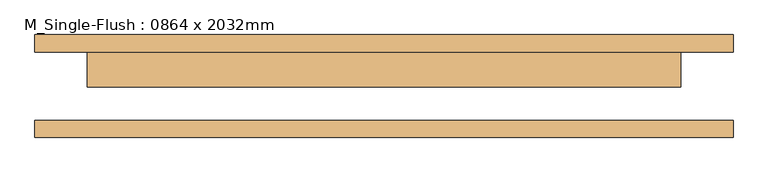
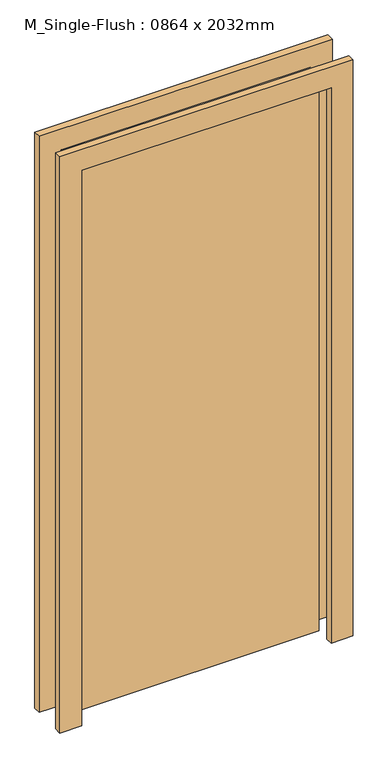
"""IFC4 building model written with IfcOpenShell, lengths in millimetres: door geometry, M_Single-Flush : 0864 x 2032mm."""

import ifcopenshell
import ifcopenshell.guid

model = None  # the IFC model being written
_history = None  # IfcOwnerHistory: only IFC2X3 demands one
_inside = {}  # id of a spatial element -> (the spatial element, [elements in it])
_under = {}  # id of a project, library or spatial element -> (it, [spatial elements below it])
_declared = {}  # id of a project -> (the project, [libraries it declares])
_typed = {}  # id of a type object -> (the type object, [elements of that type])
_made_of = {}  # id of a material, layer set ... -> (it, [elements and type objects made of it])


def new_model(schema):
    """Start an empty IFC model of exactly this schema.

    Asked for "IFC4X3", IfcOpenShell would pick the latest addendum, in which some entities
    have other attributes; the version numbers below select the first issue.
    IFC2X3 requires an IfcOwnerHistory on every rooted entity: one is made here for all.
    """
    global model, _history
    if schema == "IFC4X3":
        model = ifcopenshell.file(schema_version=(4, 3, 0, 0))
    else:
        model = ifcopenshell.file(schema=schema)
    _inside.clear()
    _under.clear()
    _declared.clear()
    _typed.clear()
    _made_of.clear()
    _history = None
    if model.schema == "IFC2X3":
        org = make("IfcOrganization", Name="unknown")
        user = make(
            "IfcPersonAndOrganization",
            ThePerson=make("IfcPerson", FamilyName="unknown"),
            TheOrganization=org,
        )
        app = make(
            "IfcApplication",
            ApplicationDeveloper=org,
            Version="unknown",
            ApplicationFullName="unknown",
            ApplicationIdentifier="unknown",
        )
        _history = make(
            "IfcOwnerHistory",
            OwningUser=user,
            OwningApplication=app,
            ChangeAction="ADDED",
            CreationDate=0,
        )
    return model


def make(cls, **values):
    """One entity of the class cls with the attributes given. An attribute that is None is left unset."""
    return model.create_entity(
        cls, **{name: value for name, value in values.items() if value is not None}
    )


def rooted(cls, **values):
    """An entity with a GlobalId (a new one), such as an element, a storey or a relation."""
    return make(cls, GlobalId=ifcopenshell.guid.new(), OwnerHistory=_history, **values)


def si_unit(unit_type, name, prefix=None):
    """IfcSIUnit, for example si_unit("LENGTHUNIT", "METRE", prefix="MILLI")."""
    return make("IfcSIUnit", UnitType=unit_type, Prefix=prefix, Name=name)


def assignment(units):
    """IfcUnitAssignment: the units of a project."""
    return None if units is None else make("IfcUnitAssignment", Units=units)


def point(xyz):
    """IfcCartesianPoint."""
    return None if xyz is None else make("IfcCartesianPoint", Coordinates=xyz)


def direction(xyz):
    """IfcDirection."""
    return None if xyz is None else make("IfcDirection", DirectionRatios=xyz)


def frame(location, z_axis=None, x_axis=None):
    """IfcAxis2Placement3D, a coordinate frame: its origin and axes. An axis left out is left unset."""
    return make(
        "IfcAxis2Placement3D",
        Location=point(location),
        Axis=direction(z_axis),
        RefDirection=direction(x_axis),
    )


def origin():
    """The frame at (0, 0, 0) with its axes left unset."""
    return frame((0.0, 0.0, 0.0))


def origin_with_axes():
    """The frame at (0, 0, 0) with the z axis (0, 0, 1) and the x axis (1, 0, 0) written out."""
    return frame((0.0, 0.0, 0.0), z_axis=(0.0, 0.0, 1.0), x_axis=(1.0, 0.0, 0.0))


def place(relative_to, where):
    """IfcLocalPlacement: puts the frame where relative to a parent placement (None: the world)."""
    return make(
        "IfcLocalPlacement", PlacementRelTo=relative_to, RelativePlacement=where
    )


def context(
    kind, dimensions, precision=None, world=None, true_north=None, identifier=None
):
    """IfcGeometricRepresentationContext, for example the 3D "Model" context."""
    return make(
        "IfcGeometricRepresentationContext",
        ContextIdentifier=identifier,
        ContextType=kind,
        CoordinateSpaceDimension=dimensions,
        Precision=precision,
        WorldCoordinateSystem=world,
        TrueNorth=true_north,
    )


def project(units=None, contexts=None):
    """IfcProject with its units and contexts."""
    return rooted(
        "IfcProject",
        Name="project",
        RepresentationContexts=contexts,
        UnitsInContext=assignment(units),
    )


def spatial(cls, under=None, at=None, **own):
    """A site, building, storey or space (cls), placed at a placement, below another one or the project."""
    s = rooted(cls, ObjectPlacement=at, **own)
    if under is not None:
        _under.setdefault(under.id(), (under, []))[1].append(s)
    return s


def polyline(points):
    """IfcPolyline through the points."""
    return make("IfcPolyline", Points=[point(p) for p in points])


def outline(outer, holes=None, kind="AREA"):
    """IfcArbitraryClosedProfileDef: a profile drawn as a closed curve; with holes, ...WithVoids."""
    if holes is None:
        return make("IfcArbitraryClosedProfileDef", ProfileType=kind, OuterCurve=outer)
    return make(
        "IfcArbitraryProfileDefWithVoids",
        ProfileType=kind,
        OuterCurve=outer,
        InnerCurves=holes,
    )


def extrude(swept, where, along, depth):
    """IfcExtrudedAreaSolid: the profile swept, set in the frame where, extruded along a direction by depth."""
    return make(
        "IfcExtrudedAreaSolid",
        SweptArea=swept,
        Position=where,
        ExtrudedDirection=direction(along),
        Depth=depth,
    )


def shape(context_of_items, identifier, shape_type, items):
    """IfcShapeRepresentation: the items that make up one representation, for example the "Body"."""
    return make(
        "IfcShapeRepresentation",
        ContextOfItems=context_of_items,
        RepresentationIdentifier=identifier,
        RepresentationType=shape_type,
        Items=items,
    )


def source(mapping_origin, context_of_items, identifier, shape_type, items):
    """IfcRepresentationMap: a shape defined once, which mapped items show again and again."""
    return make(
        "IfcRepresentationMap",
        MappingOrigin=mapping_origin,
        MappedRepresentation=shape(context_of_items, identifier, shape_type, items),
    )


def transform(
    local_origin,
    x_axis=None,
    y_axis=None,
    z_axis=None,
    scale=None,
    scale2=None,
    scale3=None,
    uniform=True,
):
    """IfcCartesianTransformationOperator3D, or its non-uniform kind. x_axis, y_axis, z_axis: its Axis1, 2, 3."""
    if uniform:
        return make(
            "IfcCartesianTransformationOperator3D",
            Axis1=direction(x_axis),
            Axis2=direction(y_axis),
            LocalOrigin=point(local_origin),
            Scale=scale,
            Axis3=direction(z_axis),
        )
    return make(
        "IfcCartesianTransformationOperator3DnonUniform",
        Axis1=direction(x_axis),
        Axis2=direction(y_axis),
        LocalOrigin=point(local_origin),
        Scale=scale,
        Axis3=direction(z_axis),
        Scale2=scale2,
        Scale3=scale3,
    )


def mapped(mapping_source, mapping_target):
    """IfcMappedItem: shows the shape of a source again, moved by a transform."""
    return make(
        "IfcMappedItem", MappingSource=mapping_source, MappingTarget=mapping_target
    )


def made_of(thing, what):
    """Note that an element or type object is made of a material, layer set ...; save() writes the relation."""
    if what is not None:
        _made_of.setdefault(what.id(), (what, []))[1].append(thing)
    return thing


def element(
    cls,
    number,
    at=None,
    inside=None,
    cuts=None,
    type_object=None,
    material=None,
    context=None,
    identifier="Body",
    shape_type=None,
    held_by="IfcProductDefinitionShape",
    body=None,
    shapes=None,
    **own,
):
    """One element of the class cls, such as IfcWall. Its Tag is "e" and its number.

    at: its placement. inside: the storey or other place that contains it. cuts: it is an
    opening in that element (IfcRelVoidsElement). A single representation is given by context,
    identifier, shape_type and body (its items); several are given by shapes. held_by: the class
    of the entity that holds the representations. save() writes the other relations.
    """
    e = rooted(cls, Tag="e%d" % number, ObjectPlacement=at, **own)
    if body is not None:
        shapes = [shape(context, identifier, shape_type, body)]
    if shapes is not None:
        e.Representation = make(held_by, Representations=shapes)
    if inside is not None:
        _inside.setdefault(inside.id(), (inside, []))[1].append(e)
    if cuts is not None:
        rooted(
            "IfcRelVoidsElement", RelatingBuildingElement=cuts, RelatedOpeningElement=e
        )
    if type_object is not None:
        _typed.setdefault(type_object.id(), (type_object, []))[1].append(e)
    return made_of(e, material)


def aggregate(whole, parts):
    """IfcRelAggregates: a whole, such as a stair, and the parts it consists of."""
    return rooted("IfcRelAggregates", RelatingObject=whole, RelatedObjects=parts)


def save(model, path):
    """Write the relations noted so far, then the file.

    IfcRelAggregates (storeys below a building ...), IfcRelContainedInSpatialStructure (elements
    in a storey), IfcRelDefinesByType, IfcRelAssociatesMaterial and IfcRelDeclares: one each for
    every whole, place, type object, material and project.
    """
    for whole, parts in _under.values():
        aggregate(whole, parts)
    for where, things in _inside.values():
        rooted(
            "IfcRelContainedInSpatialStructure",
            RelatedElements=things,
            RelatingStructure=where,
        )
    for kind, things in _typed.values():
        rooted("IfcRelDefinesByType", RelatedObjects=things, RelatingType=kind)
    for what, things in _made_of.values():
        rooted("IfcRelAssociatesMaterial", RelatedObjects=things, RelatingMaterial=what)
    for by, libraries in _declared.values():
        rooted("IfcRelDeclares", RelatingContext=by, RelatedDefinitions=libraries)
    model.write(path)


def m_single_flush_0864_x_2032mm_252f296b(model_context):
    return source(origin(), model_context, "Body", "SweptSolid", [
        extrude(outline(polyline([(2108.0, -508.0), (0.0, -508.0), (0.0, -432.0), (2032.0, -432.0), (2032.0, 432.0), (0.0, 432.0), (0.0, 508.0), (2108.0, 508.0), (2108.0, -508.0)])), frame((0.0, 50.0, 0.0), z_axis=(0.0, 1.0, 0.0), x_axis=(0.0, 0.0, 1.0)), (0.0, 0.0, 1.0), 25.0),
        extrude(outline(polyline([(2108.0, 508.0), (2108.0, -508.0), (0.0, -508.0), (0.0, -432.0), (2032.0, -432.0), (2032.0, 432.0), (0.0, 432.0), (0.0, 508.0), (2108.0, 508.0)])), frame((0.0, -75.0, 0.0), z_axis=(0.0, 1.0, 0.0), x_axis=(0.0, 0.0, 1.0)), (0.0, 0.0, 1.0), 25.0),
        extrude(outline(polyline([(432.0, -1.0), (-432.0, -1.0), (-432.0, 50.0), (432.0, 50.0), (432.0, -1.0)])), origin_with_axes(), (0.0, 0.0, 1.0), 2032.0),
    ])


if __name__ == "__main__":
    model = new_model("IFC4")
    model_context = context("Model", 3, world=origin())
    ifc_project = project(units=[si_unit("LENGTHUNIT", "METRE", prefix="MILLI")], contexts=[model_context])
    site = spatial("IfcSite", under=ifc_project)
    building = spatial("IfcBuilding", under=site)
    placement = place(None, origin())
    m_single_flush_0864_x_2032mm_shape = m_single_flush_0864_x_2032mm_252f296b(model_context)
    element("IfcDoor", 1, ObjectType="M_Single-Flush : 0864 x 2032mm", at=placement, inside=building, context=model_context, shape_type="MappedRepresentation", body=[
        mapped(m_single_flush_0864_x_2032mm_shape, transform((0.0, 0.0, 0.0), x_axis=(1.0, 0.0, 0.0), y_axis=(0.0, 1.0, 0.0), z_axis=(0.0, 0.0, 1.0))),
    ])
    save(model, "model.ifc")

# Revit data of these elements
# Type "M_Single-Flush : 0864 x 2032mm"
#   Type Mark = "21"
#   Thickness = 5.1 cm
#   Height = 203.2 cm
#   Trim Projection Ext = 2.5 cm
#   Trim Projection Int = 2.5 cm
#   Trim Width = 7.6 cm
#   Width = 86.4 cm
#   Door Material = Door - Panel
#   Frame Material = Door - Frame
#   Function = (empty or 0)
#   Wall Closure = (empty or 0)
# Element 1 (IfcDoor, "M_Single-Flush : 0864 x 2032mm")
#   Materials on its faces: "Door - Frame", "Door - Panel"
# Materials
#   "Door - Panel": class "Wood", colour RGB 114 82 51, transparency 0
#   "Door - Frame": class "Miscellaneous", colour RGB 153 76 43, transparency 0
